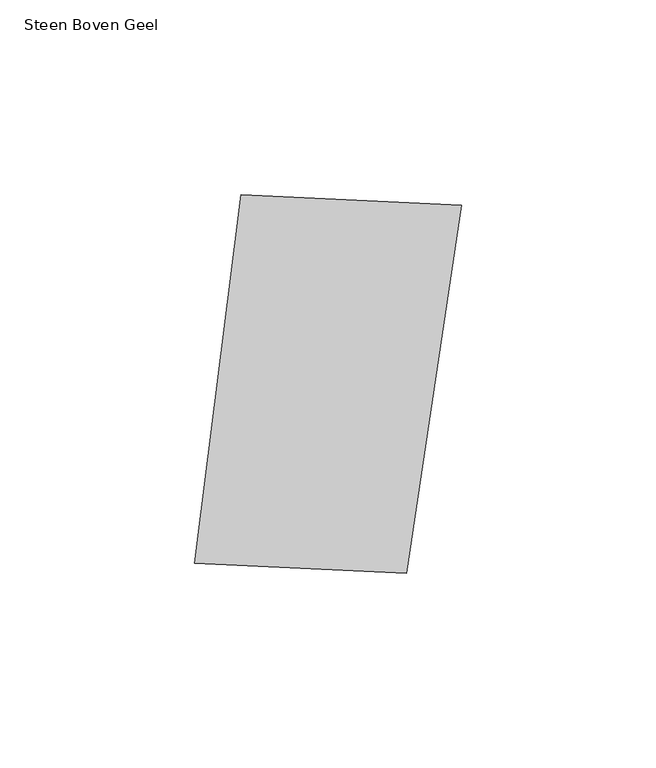
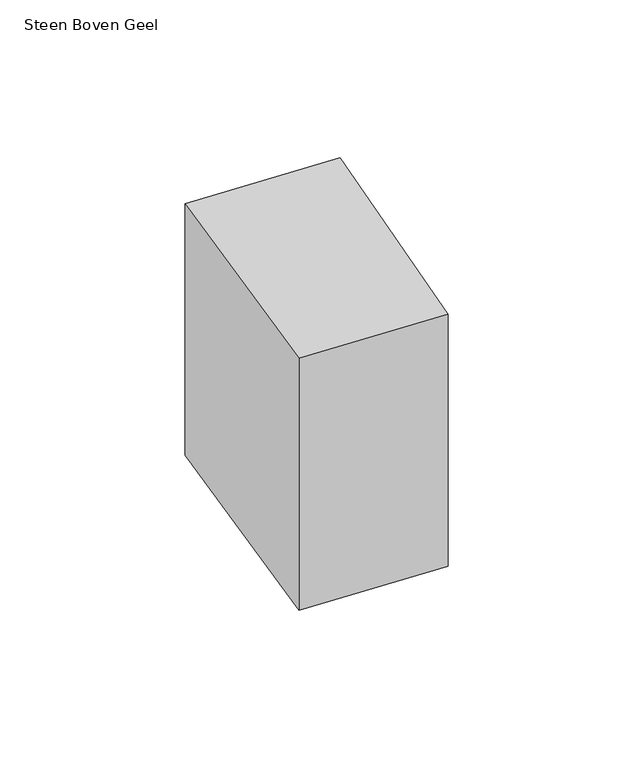
"""IFC4 building model written with IfcOpenShell, lengths in millimetres: proxy geometry, 00_GMA_steen_versie_4 : Steen Boven Geel."""

import ifcopenshell
import ifcopenshell.guid

model = None  # the IFC model being written
_history = None  # IfcOwnerHistory: only IFC2X3 demands one
_inside = {}  # id of a spatial element -> (the spatial element, [elements in it])
_under = {}  # id of a project, library or spatial element -> (it, [spatial elements below it])
_declared = {}  # id of a project -> (the project, [libraries it declares])
_typed = {}  # id of a type object -> (the type object, [elements of that type])
_made_of = {}  # id of a material, layer set ... -> (it, [elements and type objects made of it])


def new_model(schema):
    """Start an empty IFC model of exactly this schema.

    Asked for "IFC4X3", IfcOpenShell would pick the latest addendum, in which some entities
    have other attributes; the version numbers below select the first issue.
    IFC2X3 requires an IfcOwnerHistory on every rooted entity: one is made here for all.
    """
    global model, _history
    if schema == "IFC4X3":
        model = ifcopenshell.file(schema_version=(4, 3, 0, 0))
    else:
        model = ifcopenshell.file(schema=schema)
    _inside.clear()
    _under.clear()
    _declared.clear()
    _typed.clear()
    _made_of.clear()
    _history = None
    if model.schema == "IFC2X3":
        org = make("IfcOrganization", Name="unknown")
        user = make(
            "IfcPersonAndOrganization",
            ThePerson=make("IfcPerson", FamilyName="unknown"),
            TheOrganization=org,
        )
        app = make(
            "IfcApplication",
            ApplicationDeveloper=org,
            Version="unknown",
            ApplicationFullName="unknown",
            ApplicationIdentifier="unknown",
        )
        _history = make(
            "IfcOwnerHistory",
            OwningUser=user,
            OwningApplication=app,
            ChangeAction="ADDED",
            CreationDate=0,
        )
    return model


def make(cls, **values):
    """One entity of the class cls with the attributes given. An attribute that is None is left unset."""
    return model.create_entity(
        cls, **{name: value for name, value in values.items() if value is not None}
    )


def rooted(cls, **values):
    """An entity with a GlobalId (a new one), such as an element, a storey or a relation."""
    return make(cls, GlobalId=ifcopenshell.guid.new(), OwnerHistory=_history, **values)


def si_unit(unit_type, name, prefix=None):
    """IfcSIUnit, for example si_unit("LENGTHUNIT", "METRE", prefix="MILLI")."""
    return make("IfcSIUnit", UnitType=unit_type, Prefix=prefix, Name=name)


def assignment(units):
    """IfcUnitAssignment: the units of a project."""
    return None if units is None else make("IfcUnitAssignment", Units=units)


def point(xyz):
    """IfcCartesianPoint."""
    return None if xyz is None else make("IfcCartesianPoint", Coordinates=xyz)


def direction(xyz):
    """IfcDirection."""
    return None if xyz is None else make("IfcDirection", DirectionRatios=xyz)


def frame(location, z_axis=None, x_axis=None):
    """IfcAxis2Placement3D, a coordinate frame: its origin and axes. An axis left out is left unset."""
    return make(
        "IfcAxis2Placement3D",
        Location=point(location),
        Axis=direction(z_axis),
        RefDirection=direction(x_axis),
    )


def origin():
    """The frame at (0, 0, 0) with its axes left unset."""
    return frame((0.0, 0.0, 0.0))


def origin_with_axes():
    """The frame at (0, 0, 0) with the z axis (0, 0, 1) and the x axis (1, 0, 0) written out."""
    return frame((0.0, 0.0, 0.0), z_axis=(0.0, 0.0, 1.0), x_axis=(1.0, 0.0, 0.0))


def place(relative_to, where):
    """IfcLocalPlacement: puts the frame where relative to a parent placement (None: the world)."""
    return make(
        "IfcLocalPlacement", PlacementRelTo=relative_to, RelativePlacement=where
    )


def context(
    kind, dimensions, precision=None, world=None, true_north=None, identifier=None
):
    """IfcGeometricRepresentationContext, for example the 3D "Model" context."""
    return make(
        "IfcGeometricRepresentationContext",
        ContextIdentifier=identifier,
        ContextType=kind,
        CoordinateSpaceDimension=dimensions,
        Precision=precision,
        WorldCoordinateSystem=world,
        TrueNorth=true_north,
    )


def project(units=None, contexts=None):
    """IfcProject with its units and contexts."""
    return rooted(
        "IfcProject",
        Name="project",
        RepresentationContexts=contexts,
        UnitsInContext=assignment(units),
    )


def spatial(cls, under=None, at=None, **own):
    """A site, building, storey or space (cls), placed at a placement, below another one or the project."""
    s = rooted(cls, ObjectPlacement=at, **own)
    if under is not None:
        _under.setdefault(under.id(), (under, []))[1].append(s)
    return s


def polyline(points):
    """IfcPolyline through the points."""
    return make("IfcPolyline", Points=[point(p) for p in points])


def outline(outer, holes=None, kind="AREA"):
    """IfcArbitraryClosedProfileDef: a profile drawn as a closed curve; with holes, ...WithVoids."""
    if holes is None:
        return make("IfcArbitraryClosedProfileDef", ProfileType=kind, OuterCurve=outer)
    return make(
        "IfcArbitraryProfileDefWithVoids",
        ProfileType=kind,
        OuterCurve=outer,
        InnerCurves=holes,
    )


def extrude(swept, where, along, depth):
    """IfcExtrudedAreaSolid: the profile swept, set in the frame where, extruded along a direction by depth."""
    return make(
        "IfcExtrudedAreaSolid",
        SweptArea=swept,
        Position=where,
        ExtrudedDirection=direction(along),
        Depth=depth,
    )


def shape(context_of_items, identifier, shape_type, items):
    """IfcShapeRepresentation: the items that make up one representation, for example the "Body"."""
    return make(
        "IfcShapeRepresentation",
        ContextOfItems=context_of_items,
        RepresentationIdentifier=identifier,
        RepresentationType=shape_type,
        Items=items,
    )


def source(mapping_origin, context_of_items, identifier, shape_type, items):
    """IfcRepresentationMap: a shape defined once, which mapped items show again and again."""
    return make(
        "IfcRepresentationMap",
        MappingOrigin=mapping_origin,
        MappedRepresentation=shape(context_of_items, identifier, shape_type, items),
    )


def transform(
    local_origin,
    x_axis=None,
    y_axis=None,
    z_axis=None,
    scale=None,
    scale2=None,
    scale3=None,
    uniform=True,
):
    """IfcCartesianTransformationOperator3D, or its non-uniform kind. x_axis, y_axis, z_axis: its Axis1, 2, 3."""
    if uniform:
        return make(
            "IfcCartesianTransformationOperator3D",
            Axis1=direction(x_axis),
            Axis2=direction(y_axis),
            LocalOrigin=point(local_origin),
            Scale=scale,
            Axis3=direction(z_axis),
        )
    return make(
        "IfcCartesianTransformationOperator3DnonUniform",
        Axis1=direction(x_axis),
        Axis2=direction(y_axis),
        LocalOrigin=point(local_origin),
        Scale=scale,
        Axis3=direction(z_axis),
        Scale2=scale2,
        Scale3=scale3,
    )


def mapped(mapping_source, mapping_target):
    """IfcMappedItem: shows the shape of a source again, moved by a transform."""
    return make(
        "IfcMappedItem", MappingSource=mapping_source, MappingTarget=mapping_target
    )


def made_of(thing, what):
    """Note that an element or type object is made of a material, layer set ...; save() writes the relation."""
    if what is not None:
        _made_of.setdefault(what.id(), (what, []))[1].append(thing)
    return thing


def element(
    cls,
    number,
    at=None,
    inside=None,
    cuts=None,
    type_object=None,
    material=None,
    context=None,
    identifier="Body",
    shape_type=None,
    held_by="IfcProductDefinitionShape",
    body=None,
    shapes=None,
    **own,
):
    """One element of the class cls, such as IfcWall. Its Tag is "e" and its number.

    at: its placement. inside: the storey or other place that contains it. cuts: it is an
    opening in that element (IfcRelVoidsElement). A single representation is given by context,
    identifier, shape_type and body (its items); several are given by shapes. held_by: the class
    of the entity that holds the representations. save() writes the other relations.
    """
    e = rooted(cls, Tag="e%d" % number, ObjectPlacement=at, **own)
    if body is not None:
        shapes = [shape(context, identifier, shape_type, body)]
    if shapes is not None:
        e.Representation = make(held_by, Representations=shapes)
    if inside is not None:
        _inside.setdefault(inside.id(), (inside, []))[1].append(e)
    if cuts is not None:
        rooted(
            "IfcRelVoidsElement", RelatingBuildingElement=cuts, RelatedOpeningElement=e
        )
    if type_object is not None:
        _typed.setdefault(type_object.id(), (type_object, []))[1].append(e)
    return made_of(e, material)


def aggregate(whole, parts):
    """IfcRelAggregates: a whole, such as a stair, and the parts it consists of."""
    return rooted("IfcRelAggregates", RelatingObject=whole, RelatedObjects=parts)


def save(model, path):
    """Write the relations noted so far, then the file.

    IfcRelAggregates (storeys below a building ...), IfcRelContainedInSpatialStructure (elements
    in a storey), IfcRelDefinesByType, IfcRelAssociatesMaterial and IfcRelDeclares: one each for
    every whole, place, type object, material and project.
    """
    for whole, parts in _under.values():
        aggregate(whole, parts)
    for where, things in _inside.values():
        rooted(
            "IfcRelContainedInSpatialStructure",
            RelatedElements=things,
            RelatingStructure=where,
        )
    for kind, things in _typed.values():
        rooted("IfcRelDefinesByType", RelatedObjects=things, RelatingType=kind)
    for what, things in _made_of.values():
        rooted("IfcRelAssociatesMaterial", RelatedObjects=things, RelatingMaterial=what)
    for by, libraries in _declared.values():
        rooted("IfcRelDeclares", RelatingContext=by, RelatedDefinitions=libraries)
    model.write(path)


def steen_boven_geel_fc8a2ba8(model_context):
    return source(origin(), model_context, "Body", "SweptSolid", [
        extrude(outline(polyline([(107.9390236, 118.5393411), (93.9130218, 24.0769673), (39.4213154, 26.6884171), (51.3369085, 121.2433534), (107.9390236, 118.5393411)])), origin_with_axes(), (0.0, 0.0, 1.0), 100.0),
    ])


if __name__ == "__main__":
    model = new_model("IFC4")
    model_context = context("Model", 3, world=origin())
    ifc_project = project(units=[si_unit("LENGTHUNIT", "METRE", prefix="MILLI")], contexts=[model_context])
    site = spatial("IfcSite", under=ifc_project)
    building = spatial("IfcBuilding", under=site)
    placement = place(None, origin())
    steen_boven_geel_shape = steen_boven_geel_fc8a2ba8(model_context)
    element("IfcBuildingElementProxy", 1, Name="00_GMA_steen_versie_4 : Steen Boven Geel", ObjectType="00_GMA_steen_versie_4 : Steen Boven Geel", at=placement, inside=building, context=model_context, shape_type="MappedRepresentation", body=[
        mapped(steen_boven_geel_shape, transform((0.0, 0.0, 0.0), x_axis=(1.0, 0.0, 0.0), y_axis=(0.0, 1.0, 0.0), z_axis=(0.0, 0.0, 1.0))),
    ])
    save(model, "model.ifc")

# Revit data of these elements
# Type "00_GMA_steen_versie_4 : Steen Boven Geel"
#   StootVoegHalfBoven [instance default] = 5 mm
#   StootVoegHalf [instance default] = 5 mm
#   StootVoegBreedteOnder = 10 mm
#   StootVoegBreedteBoven = 10 mm
#   Steendikte = 100 mm
#   LintVoegOnderHalf = 5 mm
#   LintVoegOnder = 10 mm
#   LintVoegBovenHalf = 0 mm
#   LintVoegBoven = 0 mm
#   materiaal = 21_steen_geel
#   MateriaalVoeg = none
#   Default Elevation = 0
# Element 1 (IfcBuildingElementProxy, "00_GMA_steen_versie_4 : Steen Boven Geel")
#   Materials on its faces: "21_steen_geel"
# Materials
#   "21_steen_geel": class "Unassigned", colour RGB 202 202 0, transparency 0, Cost = 0
